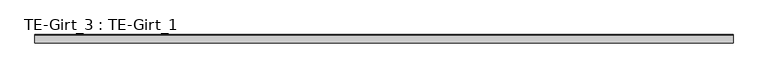
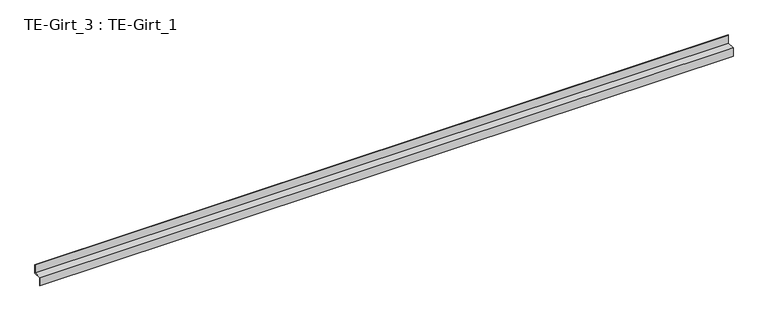
"""IFC4 building model written with IfcOpenShell, lengths in millimetres: proxy geometry, TE-Girt_3 : TE-Girt_1."""

from ifc_helpers import new_model, si_unit, frame, origin, place, context, project, spatial, polyline, outline, extrude, source, transform, mapped, element, save


def te_girt_3_te_girt_1_cbbea95c(model_context):
    return source(origin(), model_context, "Body", "SweptSolid", [
        extrude(outline(polyline([(-531639.2163841, 2374.9), (-531673.231966, 2374.9), (-531673.231966, 2337.6929688), (-531674.1249348, 2337.6929688), (-531674.1249348, 2375.7929688), (-531640.1093528, 2375.7929688), (-531640.1093528, 2413.0), (-531639.2163841, 2413.0), (-531639.2163841, 2374.9)])), frame((587365.3854739, 0.0, 0.0), z_axis=(1.0, 0.0, 0.0), x_axis=(0.0, 1.0, 0.0)), (0.0, 0.0, 1.0), 2953.258),
    ])


if __name__ == "__main__":
    model = new_model("IFC4")
    model_context = context("Model", 3, world=origin())
    ifc_project = project(units=[si_unit("LENGTHUNIT", "METRE", prefix="MILLI")], contexts=[model_context])
    site = spatial("IfcSite", under=ifc_project)
    building = spatial("IfcBuilding", under=site)
    placement = place(None, origin())
    te_girt_3_te_girt_1_shape = te_girt_3_te_girt_1_cbbea95c(model_context)
    element("IfcBuildingElementProxy", 1, Name="TE-Girt_3 : TE-Girt_1", ObjectType="TE-Girt_3 : TE-Girt_1", at=placement, inside=building, context=model_context, shape_type="MappedRepresentation", body=[
        mapped(te_girt_3_te_girt_1_shape, transform((0.0, 0.0, 0.0), x_axis=(1.0, 0.0, 0.0), y_axis=(0.0, 1.0, 0.0), z_axis=(0.0, 0.0, 1.0))),
    ])
    save(model, "model.ifc")

# Revit data of these elements
# Element 1 (IfcBuildingElementProxy, "TE-Girt_3 : TE-Girt_1")
#   Materials on its faces: "Z-FURRING, COLD-FORMED GALV."
# Materials
#   "Z-FURRING, COLD-FORMED GALV.": class "Generic", colour RGB 143 142 141, transparency 0, Cost = 0
